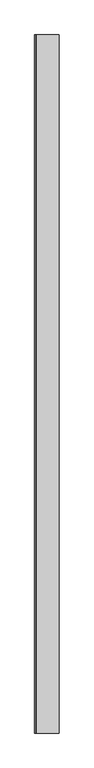
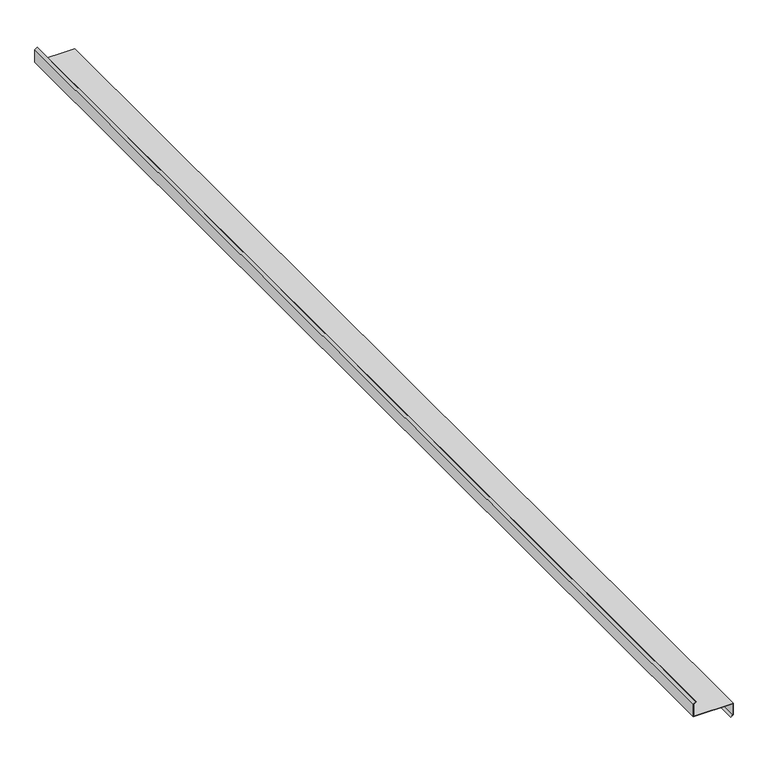
"""IFC4 building model written with IfcOpenShell, lengths in millimetres: proxy geometry, Generic Models 7:Generic Models 1:1:Generic Models 1:1 : Generic Models 7:Generic Models 1:337419:39 : Generic Models 7:Generic Models 1:1:Generic Models 1:1 : Generic Models 7:Generic Models 1:337419:306201."""

from ifc_helpers import new_model, si_unit, frame, origin, place, context, project, spatial, polyline, outline, extrude, source, transform, mapped, element, save


def generic_models_6c4367c0(model_context):
    return source(origin(), model_context, "Body", "SweptSolid", [
        extrude(outline(polyline([(3588.1924559, 667530.7466425), (3586.2205211, 667532.7185773), (3598.465625, 667547.3117239), (3677.8406249, 667547.3117239), (3677.8406249, 667296.0898489), (3759.492039, 667296.0898489), (3770.9044367, 667309.6906149), (3773.0326039, 667307.9048706), (3760.7874999, 667293.3117239), (3675.0624999, 667293.3117239), (3675.0624999, 667544.533599), (3599.761086, 667544.533599), (3588.1924559, 667530.7466425)])), frame((0.0, -571923.6163841, 0.0), z_axis=(0.0, 1.0, 0.0), x_axis=(0.0, 0.0, 1.0)), (0.0, 0.0, 1.0), 7315.2),
    ])


if __name__ == "__main__":
    model = new_model("IFC4")
    model_context = context("Model", 3, world=origin())
    ifc_project = project(units=[si_unit("LENGTHUNIT", "METRE", prefix="MILLI")], contexts=[model_context])
    site = spatial("IfcSite", under=ifc_project)
    building = spatial("IfcBuilding", under=site)
    placement = place(None, origin())
    generic_models_shape = generic_models_6c4367c0(model_context)
    element("IfcBuildingElementProxy", 1, Name="Generic Models 7:Generic Models 1:1:Generic Models 1:1 : Generic Models 7:Generic Models 1:337419:39 : Generic Models 7:Generic Models 1:1:Generic Models 1:1 : Generic Models 7:Generic Models 1:337419:306201", ObjectType="Generic Models 7:Generic Models 1:1:Generic Models 1:1 : Generic Models 7:Generic Models 1:337419:39 : Generic Models 7:Generic Models 1:1:Generic Models 1:1 : Generic Models 7:Generic Models 1:337419:306201", at=placement, inside=building, context=model_context, shape_type="MappedRepresentation", body=[
        mapped(generic_models_shape, transform((0.0, 0.0, 0.0), x_axis=(1.0, 0.0, 0.0), y_axis=(0.0, 1.0, 0.0), z_axis=(0.0, 0.0, 1.0))),
    ])
    save(model, "model.ifc")

# Revit data of these elements
# Type "Generic Models 7:Generic Models 1:1:Generic Models 1:1 : Generic Models 7:Generic Models 1:337419:39 : Generic Models 7:Generic Models 1:1:Generic Models 1:1 : Generic Models 7:Generic Models 1:337419:306201"
#   NameOverride = "Generic Models 7:Generic Models 1:1:Generic Models 1:1 : Generic Models 7:Generic Models 1:337419:306201"
#   ObjectTypeOverride = "Generic Models 1:1 : Generic Models 7:Generic Models 1:337419"
#   Reference = "Generic Models 1"
#   Tag = "306201"
# Element 1 (IfcBuildingElementProxy, "Generic Models 7:Generic Models 1:1:Generic Models 1:1 : Generic Models 7:Generic Models 1:337419:39 : Generic Models 7:Generic Models 1:1:Generic Models 1:1 : Generic Models 7:Generic Models 1:337419:306201")
#   Materials on its faces: "CEE' SECTION (8.0x3.5C - SEE STRUCT. DWGS)"
# Materials
#   "CEE' SECTION (8.0x3.5C - SEE STRUCT. DWGS)": class "Unassigned", colour RGB 210 209 208, transparency 0, Keynote = "M05121300.02", Cost = 0
